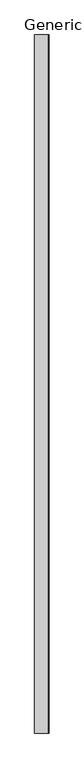
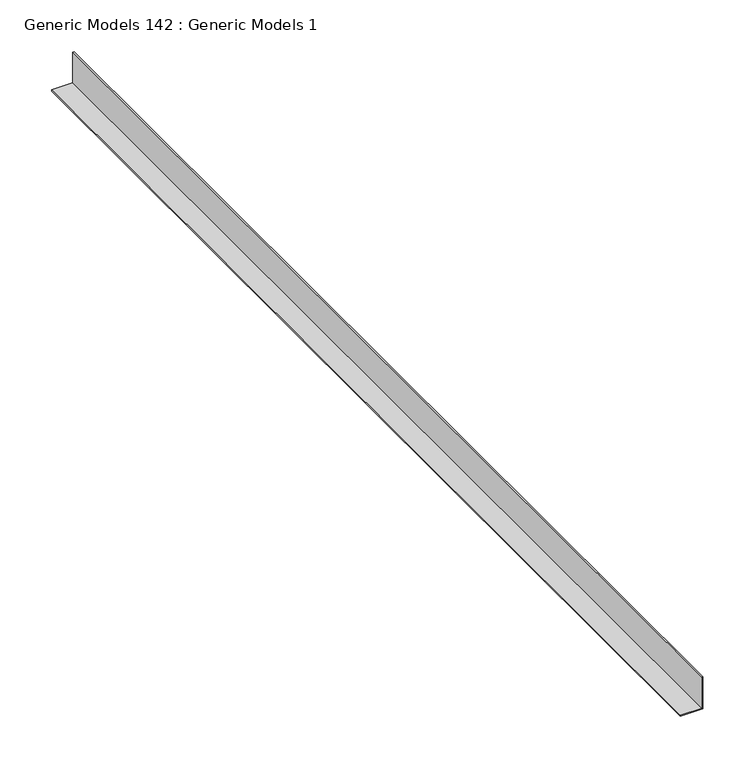
"""IFC4 building model written with IfcOpenShell, lengths in millimetres: proxy geometry, Generic Models 142 : Generic Models 1."""

import ifcopenshell
import ifcopenshell.guid

model = None  # the IFC model being written
_history = None  # IfcOwnerHistory: only IFC2X3 demands one
_inside = {}  # id of a spatial element -> (the spatial element, [elements in it])
_under = {}  # id of a project, library or spatial element -> (it, [spatial elements below it])
_declared = {}  # id of a project -> (the project, [libraries it declares])
_typed = {}  # id of a type object -> (the type object, [elements of that type])
_made_of = {}  # id of a material, layer set ... -> (it, [elements and type objects made of it])


def new_model(schema):
    """Start an empty IFC model of exactly this schema.

    Asked for "IFC4X3", IfcOpenShell would pick the latest addendum, in which some entities
    have other attributes; the version numbers below select the first issue.
    IFC2X3 requires an IfcOwnerHistory on every rooted entity: one is made here for all.
    """
    global model, _history
    if schema == "IFC4X3":
        model = ifcopenshell.file(schema_version=(4, 3, 0, 0))
    else:
        model = ifcopenshell.file(schema=schema)
    _inside.clear()
    _under.clear()
    _declared.clear()
    _typed.clear()
    _made_of.clear()
    _history = None
    if model.schema == "IFC2X3":
        org = make("IfcOrganization", Name="unknown")
        user = make(
            "IfcPersonAndOrganization",
            ThePerson=make("IfcPerson", FamilyName="unknown"),
            TheOrganization=org,
        )
        app = make(
            "IfcApplication",
            ApplicationDeveloper=org,
            Version="unknown",
            ApplicationFullName="unknown",
            ApplicationIdentifier="unknown",
        )
        _history = make(
            "IfcOwnerHistory",
            OwningUser=user,
            OwningApplication=app,
            ChangeAction="ADDED",
            CreationDate=0,
        )
    return model


def make(cls, **values):
    """One entity of the class cls with the attributes given. An attribute that is None is left unset."""
    return model.create_entity(
        cls, **{name: value for name, value in values.items() if value is not None}
    )


def rooted(cls, **values):
    """An entity with a GlobalId (a new one), such as an element, a storey or a relation."""
    return make(cls, GlobalId=ifcopenshell.guid.new(), OwnerHistory=_history, **values)


def si_unit(unit_type, name, prefix=None):
    """IfcSIUnit, for example si_unit("LENGTHUNIT", "METRE", prefix="MILLI")."""
    return make("IfcSIUnit", UnitType=unit_type, Prefix=prefix, Name=name)


def assignment(units):
    """IfcUnitAssignment: the units of a project."""
    return None if units is None else make("IfcUnitAssignment", Units=units)


def point(xyz):
    """IfcCartesianPoint."""
    return None if xyz is None else make("IfcCartesianPoint", Coordinates=xyz)


def direction(xyz):
    """IfcDirection."""
    return None if xyz is None else make("IfcDirection", DirectionRatios=xyz)


def frame(location, z_axis=None, x_axis=None):
    """IfcAxis2Placement3D, a coordinate frame: its origin and axes. An axis left out is left unset."""
    return make(
        "IfcAxis2Placement3D",
        Location=point(location),
        Axis=direction(z_axis),
        RefDirection=direction(x_axis),
    )


def origin():
    """The frame at (0, 0, 0) with its axes left unset."""
    return frame((0.0, 0.0, 0.0))


def place(relative_to, where):
    """IfcLocalPlacement: puts the frame where relative to a parent placement (None: the world)."""
    return make(
        "IfcLocalPlacement", PlacementRelTo=relative_to, RelativePlacement=where
    )


def context(
    kind, dimensions, precision=None, world=None, true_north=None, identifier=None
):
    """IfcGeometricRepresentationContext, for example the 3D "Model" context."""
    return make(
        "IfcGeometricRepresentationContext",
        ContextIdentifier=identifier,
        ContextType=kind,
        CoordinateSpaceDimension=dimensions,
        Precision=precision,
        WorldCoordinateSystem=world,
        TrueNorth=true_north,
    )


def project(units=None, contexts=None):
    """IfcProject with its units and contexts."""
    return rooted(
        "IfcProject",
        Name="project",
        RepresentationContexts=contexts,
        UnitsInContext=assignment(units),
    )


def spatial(cls, under=None, at=None, **own):
    """A site, building, storey or space (cls), placed at a placement, below another one or the project."""
    s = rooted(cls, ObjectPlacement=at, **own)
    if under is not None:
        _under.setdefault(under.id(), (under, []))[1].append(s)
    return s


def polyline(points):
    """IfcPolyline through the points."""
    return make("IfcPolyline", Points=[point(p) for p in points])


def outline(outer, holes=None, kind="AREA"):
    """IfcArbitraryClosedProfileDef: a profile drawn as a closed curve; with holes, ...WithVoids."""
    if holes is None:
        return make("IfcArbitraryClosedProfileDef", ProfileType=kind, OuterCurve=outer)
    return make(
        "IfcArbitraryProfileDefWithVoids",
        ProfileType=kind,
        OuterCurve=outer,
        InnerCurves=holes,
    )


def extrude(swept, where, along, depth):
    """IfcExtrudedAreaSolid: the profile swept, set in the frame where, extruded along a direction by depth."""
    return make(
        "IfcExtrudedAreaSolid",
        SweptArea=swept,
        Position=where,
        ExtrudedDirection=direction(along),
        Depth=depth,
    )


def shape(context_of_items, identifier, shape_type, items):
    """IfcShapeRepresentation: the items that make up one representation, for example the "Body"."""
    return make(
        "IfcShapeRepresentation",
        ContextOfItems=context_of_items,
        RepresentationIdentifier=identifier,
        RepresentationType=shape_type,
        Items=items,
    )


def source(mapping_origin, context_of_items, identifier, shape_type, items):
    """IfcRepresentationMap: a shape defined once, which mapped items show again and again."""
    return make(
        "IfcRepresentationMap",
        MappingOrigin=mapping_origin,
        MappedRepresentation=shape(context_of_items, identifier, shape_type, items),
    )


def transform(
    local_origin,
    x_axis=None,
    y_axis=None,
    z_axis=None,
    scale=None,
    scale2=None,
    scale3=None,
    uniform=True,
):
    """IfcCartesianTransformationOperator3D, or its non-uniform kind. x_axis, y_axis, z_axis: its Axis1, 2, 3."""
    if uniform:
        return make(
            "IfcCartesianTransformationOperator3D",
            Axis1=direction(x_axis),
            Axis2=direction(y_axis),
            LocalOrigin=point(local_origin),
            Scale=scale,
            Axis3=direction(z_axis),
        )
    return make(
        "IfcCartesianTransformationOperator3DnonUniform",
        Axis1=direction(x_axis),
        Axis2=direction(y_axis),
        LocalOrigin=point(local_origin),
        Scale=scale,
        Axis3=direction(z_axis),
        Scale2=scale2,
        Scale3=scale3,
    )


def mapped(mapping_source, mapping_target):
    """IfcMappedItem: shows the shape of a source again, moved by a transform."""
    return make(
        "IfcMappedItem", MappingSource=mapping_source, MappingTarget=mapping_target
    )


def made_of(thing, what):
    """Note that an element or type object is made of a material, layer set ...; save() writes the relation."""
    if what is not None:
        _made_of.setdefault(what.id(), (what, []))[1].append(thing)
    return thing


def element(
    cls,
    number,
    at=None,
    inside=None,
    cuts=None,
    type_object=None,
    material=None,
    context=None,
    identifier="Body",
    shape_type=None,
    held_by="IfcProductDefinitionShape",
    body=None,
    shapes=None,
    **own,
):
    """One element of the class cls, such as IfcWall. Its Tag is "e" and its number.

    at: its placement. inside: the storey or other place that contains it. cuts: it is an
    opening in that element (IfcRelVoidsElement). A single representation is given by context,
    identifier, shape_type and body (its items); several are given by shapes. held_by: the class
    of the entity that holds the representations. save() writes the other relations.
    """
    e = rooted(cls, Tag="e%d" % number, ObjectPlacement=at, **own)
    if body is not None:
        shapes = [shape(context, identifier, shape_type, body)]
    if shapes is not None:
        e.Representation = make(held_by, Representations=shapes)
    if inside is not None:
        _inside.setdefault(inside.id(), (inside, []))[1].append(e)
    if cuts is not None:
        rooted(
            "IfcRelVoidsElement", RelatingBuildingElement=cuts, RelatedOpeningElement=e
        )
    if type_object is not None:
        _typed.setdefault(type_object.id(), (type_object, []))[1].append(e)
    return made_of(e, material)


def aggregate(whole, parts):
    """IfcRelAggregates: a whole, such as a stair, and the parts it consists of."""
    return rooted("IfcRelAggregates", RelatingObject=whole, RelatedObjects=parts)


def save(model, path):
    """Write the relations noted so far, then the file.

    IfcRelAggregates (storeys below a building ...), IfcRelContainedInSpatialStructure (elements
    in a storey), IfcRelDefinesByType, IfcRelAssociatesMaterial and IfcRelDeclares: one each for
    every whole, place, type object, material and project.
    """
    for whole, parts in _under.values():
        aggregate(whole, parts)
    for where, things in _inside.values():
        rooted(
            "IfcRelContainedInSpatialStructure",
            RelatedElements=things,
            RelatingStructure=where,
        )
    for kind, things in _typed.values():
        rooted("IfcRelDefinesByType", RelatedObjects=things, RelatingType=kind)
    for what, things in _made_of.values():
        rooted("IfcRelAssociatesMaterial", RelatedObjects=things, RelatingMaterial=what)
    for by, libraries in _declared.values():
        rooted("IfcRelDeclares", RelatingContext=by, RelatedDefinitions=libraries)
    model.write(path)


def generic_models_142_generic_models_1_dcca0c8b(model_context):
    return source(origin(), model_context, "Body", "SweptSolid", [
        extrude(outline(polyline([(2051.1444308, 46827.9235531), (2051.1444308, 46826.3360531), (2014.6319308, 46826.3360531), (2014.6319308, 46802.5235531), (2013.0444308, 46802.5235531), (2013.0444308, 46827.9235531), (2051.1444308, 46827.9235531)])), frame((0.0, 0.0, 0.0), z_axis=(0.0, 1.0, 0.0), x_axis=(0.0, 0.0, 1.0)), (0.0, 0.0, 1.0), 1219.2),
    ])


if __name__ == "__main__":
    model = new_model("IFC4")
    model_context = context("Model", 3, world=origin())
    ifc_project = project(units=[si_unit("LENGTHUNIT", "METRE", prefix="MILLI")], contexts=[model_context])
    site = spatial("IfcSite", under=ifc_project)
    building = spatial("IfcBuilding", under=site)
    placement = place(None, origin())
    generic_models_142_generic_models_1_shape = generic_models_142_generic_models_1_dcca0c8b(model_context)
    element("IfcBuildingElementProxy", 1, Name="Generic Models 142 : Generic Models 1", ObjectType="Generic Models 142 : Generic Models 1", at=placement, inside=building, context=model_context, shape_type="MappedRepresentation", body=[
        mapped(generic_models_142_generic_models_1_shape, transform((0.0, 0.0, 0.0), x_axis=(1.0, 0.0, 0.0), y_axis=(0.0, 1.0, 0.0), z_axis=(0.0, 0.0, 1.0))),
    ])
    save(model, "model.ifc")

# Revit data of these elements
# Element 1 (IfcBuildingElementProxy, "Generic Models 142 : Generic Models 1")
#   Materials on its faces: "CEILING TRACK TO MATCH EXISTING"
# Materials
#   "CEILING TRACK TO MATCH EXISTING": class "Unassigned", colour RGB 210 209 208, transparency 0, Keynote = "M05121300.02", Cost = 0
